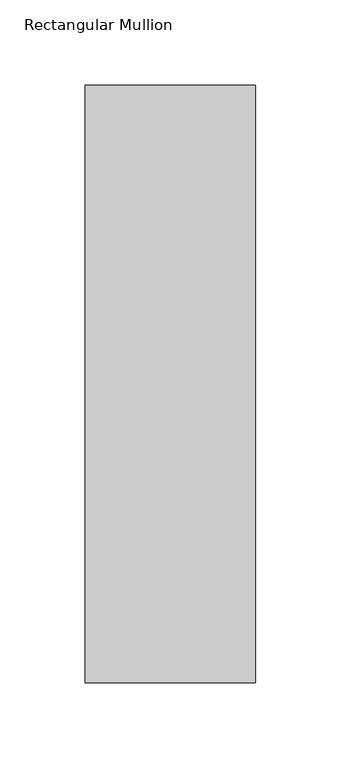
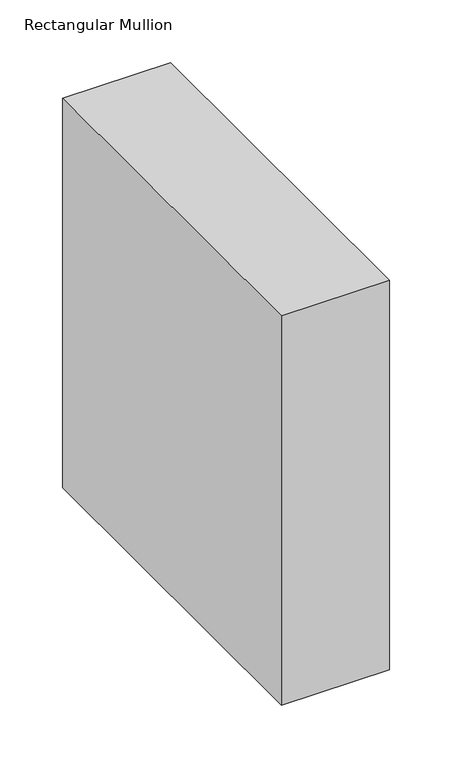
"""IFC4 building model written with IfcOpenShell, lengths in millimetres: member geometry, Rectangular Mullion : WWm-100x350-100mmOffset."""

from ifc_helpers import new_model, si_unit, frame, origin, place, context, project, spatial, polyline, outline, extrude, source, transform, mapped, element, save


def rectangular_mullion_9c918965(model_context):
    return source(origin(), model_context, "Body", "SweptSolid", [
        extrude(outline(polyline([(0.0, 175.0), (0.0, -175.0), (-100.0, -175.0), (-100.0, 175.0), (0.0, 175.0)])), frame((0.0, 0.0, -380.0), z_axis=(0.0, 0.0, 1.0), x_axis=(1.0, 0.0, 0.0)), (0.0, 0.0, 1.0), 380.0),
    ])


if __name__ == "__main__":
    model = new_model("IFC4")
    model_context = context("Model", 3, world=origin())
    ifc_project = project(units=[si_unit("LENGTHUNIT", "METRE", prefix="MILLI")], contexts=[model_context])
    site = spatial("IfcSite", under=ifc_project)
    building = spatial("IfcBuilding", under=site)
    placement = place(None, origin())
    rectangular_mullion_shape = rectangular_mullion_9c918965(model_context)
    element("IfcMember", 1, ObjectType="Rectangular Mullion : WWm-100x350-100mmOffset", at=placement, inside=building, context=model_context, shape_type="MappedRepresentation", body=[
        mapped(rectangular_mullion_shape, transform((0.0, 0.0, 0.0), x_axis=(1.0, 0.0, 0.0), y_axis=(0.0, 1.0, 0.0), z_axis=(0.0, 0.0, 1.0))),
    ])
    save(model, "model.ifc")

# Revit data of these elements
# Type "Rectangular Mullion : WWm-100x350-100mmOffset"
#   built-in parameter 1007304 = 1.14829 (stored number, unit not read)
#   built-in parameter 1007301 = 0.164042 (stored number, unit not read)
#   built-in parameter 1007300 = 0.164042 (stored number, unit not read)
# Element 1 (IfcMember, "Rectangular Mullion : WWm-100x350-100mmOffset")
#   Materials on its faces: "WW-EC-RGB-Mullion"
# Materials
#   "WW-EC-RGB-Mullion": class "Generic", colour RGB 255 255 255, transparency 0, Comments = "If region requests black mullions, switch asset color to RGB 25-25-25", Description = "Generic Color", Cost = 0
